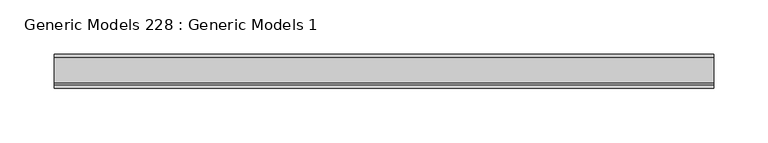
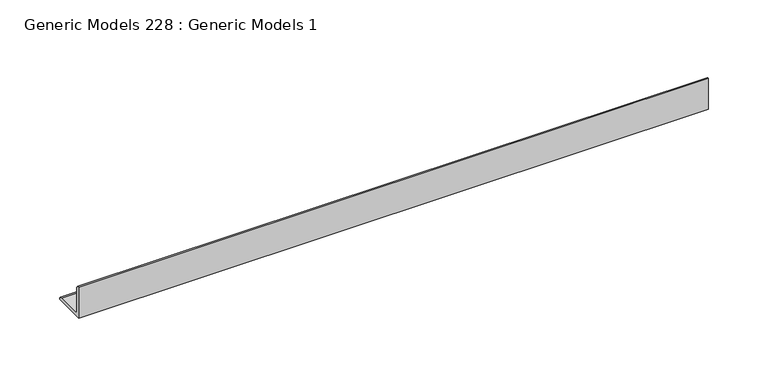
"""IFC4 building model written with IfcOpenShell, lengths in millimetres: proxy geometry, Generic Models 228 : Generic Models 1."""

from ifc_helpers import new_model, si_unit, point, frame, frame_2d, origin, place, context, project, spatial, polyline, circle_curve, trimmed, segment, composite_curve, outline, extrude, source, transform, mapped, element, save


def generic_models_228_generic_models_1_053e8907(model_context):
    return source(origin(), model_context, "Body", "SweptSolid", [
        extrude(outline(composite_curve([segment(polyline([(592.1375, 4235.45), (592.1375, 4267.2)]), True, "CONTINUOUS"), segment(trimmed(circle_curve(frame_2d((592.1375, 4264.025)), 3.175), [point((592.1375, 4267.2))], [point((595.3125, 4264.025))], False, "CARTESIAN"), True, "CONTINUOUS"), segment(polyline([(595.3125, 4264.025), (595.3125, 4240.2125)]), True, "CONTINUOUS"), segment(trimmed(circle_curve(frame_2d((596.9, 4240.2125)), 1.5875), [point((595.3125, 4240.2125))], [point((596.9, 4238.625))], True, "CARTESIAN"), True, "CONTINUOUS"), segment(polyline([(596.9, 4238.625), (620.7125, 4238.625)]), True, "CONTINUOUS"), segment(trimmed(circle_curve(frame_2d((620.7125, 4235.45)), 3.175), [point((620.7125, 4238.625))], [point((623.8875, 4235.45))], False, "CARTESIAN"), True, "CONTINUOUS"), segment(polyline([(623.8875, 4235.45), (592.1375, 4235.45)]), True, "CONTINUOUS")], self_intersect=False)), frame((46753.4625, 0.0, 0.0), z_axis=(1.0, 0.0, 0.0), x_axis=(0.0, 1.0, 0.0)), (0.0, 0.0, 1.0), 609.6),
    ])


if __name__ == "__main__":
    model = new_model("IFC4")
    model_context = context("Model", 3, world=origin())
    ifc_project = project(units=[si_unit("LENGTHUNIT", "METRE", prefix="MILLI")], contexts=[model_context])
    site = spatial("IfcSite", under=ifc_project)
    building = spatial("IfcBuilding", under=site)
    placement = place(None, origin())
    generic_models_228_generic_models_1_shape = generic_models_228_generic_models_1_053e8907(model_context)
    element("IfcBuildingElementProxy", 1, Name="Generic Models 228 : Generic Models 1", ObjectType="Generic Models 228 : Generic Models 1", at=placement, inside=building, context=model_context, shape_type="MappedRepresentation", body=[
        mapped(generic_models_228_generic_models_1_shape, transform((0.0, 0.0, 0.0), x_axis=(1.0, 0.0, 0.0), y_axis=(0.0, 1.0, 0.0), z_axis=(0.0, 0.0, 1.0))),
    ])
    save(model, "model.ifc")

# Revit data of these elements
# Element 1 (IfcBuildingElementProxy, "Generic Models 228 : Generic Models 1")
#   Materials on its faces: "BULKHEAD FRAME WORK"
# Materials
#   "BULKHEAD FRAME WORK": class "Metal", colour RGB 189 187 185, transparency 0, Description = "Structural steel 50ksi", Cost = 0
